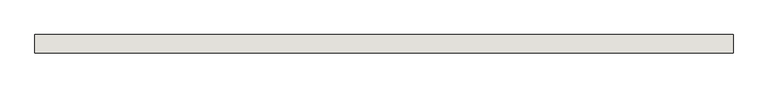
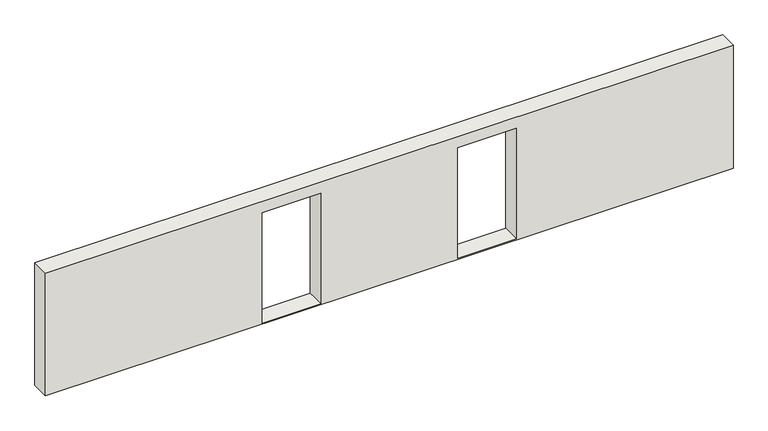
"""IFC4 building model written with IfcOpenShell, lengths in millimetres: wall geometry, 0_3d_modell."""

from ifc_helpers import new_model, si_unit, frame, origin, place, context, project, spatial, polyline, outline, extrude, source, transform, mapped, element, save


def wall_1a8f0b55(model_context):
    return source(origin(), model_context, "Body", "SweptSolid", [
        extrude(outline(polyline([(0.0, 0.0), (0.0, 13300.0), (2510.0, 13300.0), (2510.0, 0.0), (0.0, 0.0)]), holes=[polyline([(20.0, 4190.0), (2280.0, 4190.0), (2280.0, 5325.0), (20.0, 5325.0), (20.0, 4190.0)]), polyline([(20.0, 7975.0), (2280.0, 7975.0), (2280.0, 9110.0), (20.0, 9110.0), (20.0, 7975.0)])]), frame((0.0, 0.0, 0.0), z_axis=(0.0, 1.0, 0.0), x_axis=(0.0, 0.0, 1.0)), (0.0, 0.0, 1.0), 350.0),
    ])


if __name__ == "__main__":
    model = new_model("IFC4")
    model_context = context("Model", 3, world=origin())
    ifc_project = project(units=[si_unit("LENGTHUNIT", "METRE", prefix="MILLI")], contexts=[model_context])
    site = spatial("IfcSite", under=ifc_project)
    building = spatial("IfcBuilding", under=site)
    placement = place(None, origin())
    wall_shape = wall_1a8f0b55(model_context)
    element("IfcWall", 1, ObjectType="0_3d_modell", at=placement, inside=building, context=model_context, shape_type="MappedRepresentation", body=[
        mapped(wall_shape, transform((0.0, 0.0, 0.0), x_axis=(1.0, 0.0, 0.0), y_axis=(0.0, 1.0, 0.0), z_axis=(0.0, 0.0, 1.0))),
    ])
    save(model, "model.ifc")

# Revit data of these elements
# Element 1 (IfcWall, "0_3d_modell")
#   Materials on its faces: "holzschalung"
# Materials
#   "holzschalung": class "Unassigned", colour RGB 128 128 128, transparency 0
